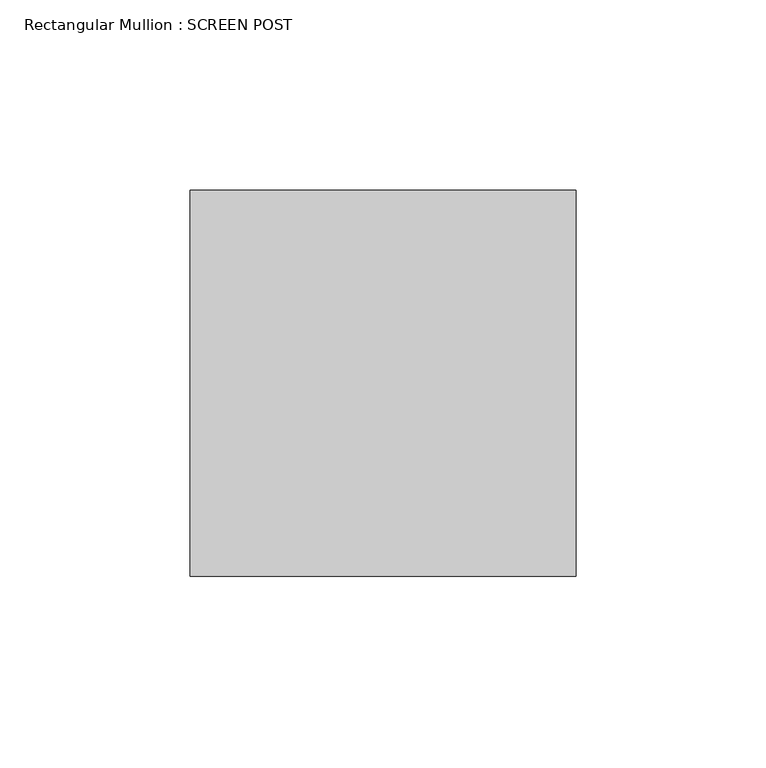
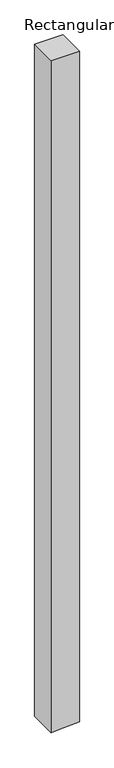
"""IFC4 building model written with IfcOpenShell, lengths in millimetres: member geometry, Rectangular Mullion : SCREEN POST."""

from ifc_helpers import new_model, si_unit, frame, origin, place, context, project, spatial, polyline, outline, extrude, source, transform, mapped, element, save


def rectangular_mullion_screen_post_2e67cbde(model_context):
    return source(origin(), model_context, "Body", "SweptSolid", [
        extrude(outline(polyline([(0.0, 50.8), (0.0, -50.8), (-2550.6632208, -50.8), (-2547.8800165, -6.3490391), (-2544.3017486, 50.8), (0.0, 50.8)])), frame((0.0, -50.8, 0.0), z_axis=(0.0, 1.0, 0.0), x_axis=(0.0, 0.0, 1.0)), (0.0, 0.0, 1.0), 101.6),
    ])


if __name__ == "__main__":
    model = new_model("IFC4")
    model_context = context("Model", 3, world=origin())
    ifc_project = project(units=[si_unit("LENGTHUNIT", "METRE", prefix="MILLI")], contexts=[model_context])
    site = spatial("IfcSite", under=ifc_project)
    building = spatial("IfcBuilding", under=site)
    placement = place(None, origin())
    rectangular_mullion_screen_post_shape = rectangular_mullion_screen_post_2e67cbde(model_context)
    element("IfcMember", 1, ObjectType="Rectangular Mullion : SCREEN POST", at=placement, inside=building, context=model_context, shape_type="MappedRepresentation", body=[
        mapped(rectangular_mullion_screen_post_shape, transform((0.0, 0.0, 0.0), x_axis=(1.0, 0.0, 0.0), y_axis=(0.0, 1.0, 0.0), z_axis=(0.0, 0.0, 1.0))),
    ])
    save(model, "model.ifc")

# Revit data of these elements
# Type "Rectangular Mullion : SCREEN POST"
#   built-in parameter 1007304 = 0.333333 (stored number, unit not read)
#   built-in parameter 1007301 = 0.166667 (stored number, unit not read)
#   built-in parameter 1007300 = 0.166667 (stored number, unit not read)
# Element 1 (IfcMember, "Rectangular Mullion : SCREEN POST")
#   Materials on its faces: "GLULAMS COLUMNS\n(PRESSURE TREATED W/ PENTA IN SOLVENT) (EXTERIOR STAIN: PENOFIN VERDE EXT. STAIN - COLOR: CEDAR)"
# Materials
#   "GLULAMS COLUMNS\n(PRESSURE TREATED W/ PENTA IN SOLVENT) (EXTERIOR STAIN: PENOFIN VERDE EXT. STAIN - COLOR: CEDAR)": class "Wood", colour RGB 164 134 123, transparency 0, Description = "Pinus Echinata", Cost = 0
